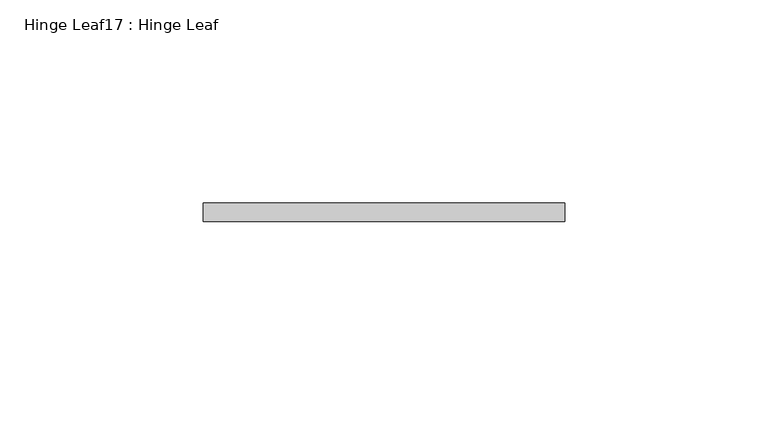
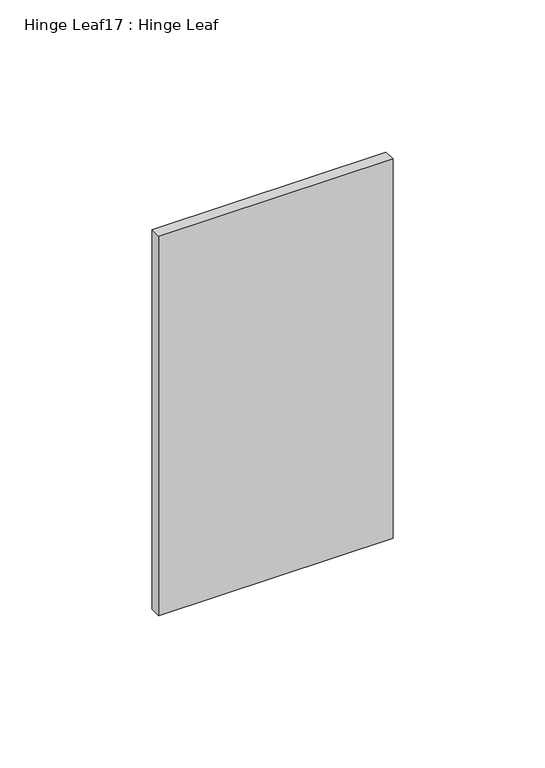
"""IFC4 building model written with IfcOpenShell, lengths in millimetres: proxy geometry, Hinge Leaf17 : Hinge Leaf."""

from ifc_helpers import new_model, si_unit, frame, origin, place, context, project, spatial, polyline, outline, extrude, source, transform, mapped, element, save


def hinge_leaf17_hinge_leaf_0c583ee0(model_context):
    return source(origin(), model_context, "Body", "SweptSolid", [
        extrude(outline(polyline([(587327.7934739, -534096.6663841), (587416.6934739, -534096.6663841), (587416.6934739, -534101.2383841), (587327.7934739, -534101.2383841), (587327.7934739, -534096.6663841)])), frame((0.0, 0.0, 1936.75), z_axis=(0.0, 0.0, 1.0), x_axis=(1.0, 0.0, 0.0)), (0.0, 0.0, 1.0), 152.4),
    ])


if __name__ == "__main__":
    model = new_model("IFC4")
    model_context = context("Model", 3, world=origin())
    ifc_project = project(units=[si_unit("LENGTHUNIT", "METRE", prefix="MILLI")], contexts=[model_context])
    site = spatial("IfcSite", under=ifc_project)
    building = spatial("IfcBuilding", under=site)
    placement = place(None, origin())
    hinge_leaf17_hinge_leaf_shape = hinge_leaf17_hinge_leaf_0c583ee0(model_context)
    element("IfcBuildingElementProxy", 1, Name="Hinge Leaf17 : Hinge Leaf", ObjectType="Hinge Leaf17 : Hinge Leaf", at=placement, inside=building, context=model_context, shape_type="MappedRepresentation", body=[
        mapped(hinge_leaf17_hinge_leaf_shape, transform((0.0, 0.0, 0.0), x_axis=(1.0, 0.0, 0.0), y_axis=(0.0, 1.0, 0.0), z_axis=(0.0, 0.0, 1.0))),
    ])
    save(model, "model.ifc")

# Revit data of these elements
# Element 1 (IfcBuildingElementProxy, "Hinge Leaf17 : Hinge Leaf")
#   Materials on its faces: "6\"X6\" WELD-ON STL BUTT HINGE"
# Materials
#   "6\"X6\" WELD-ON STL BUTT HINGE": class "Metal", colour RGB 189 187 185, transparency 0, Description = "Carbon steel", Cost = 0
